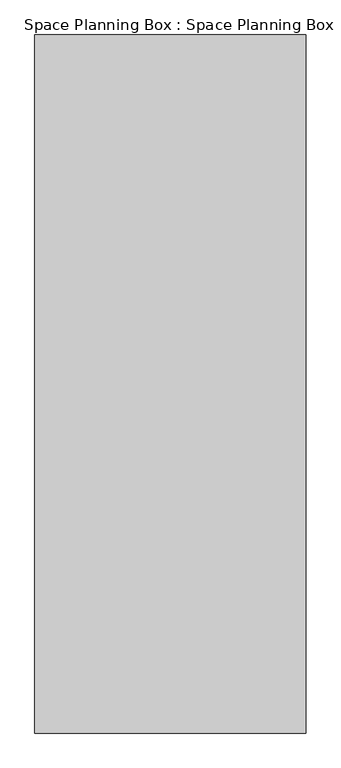
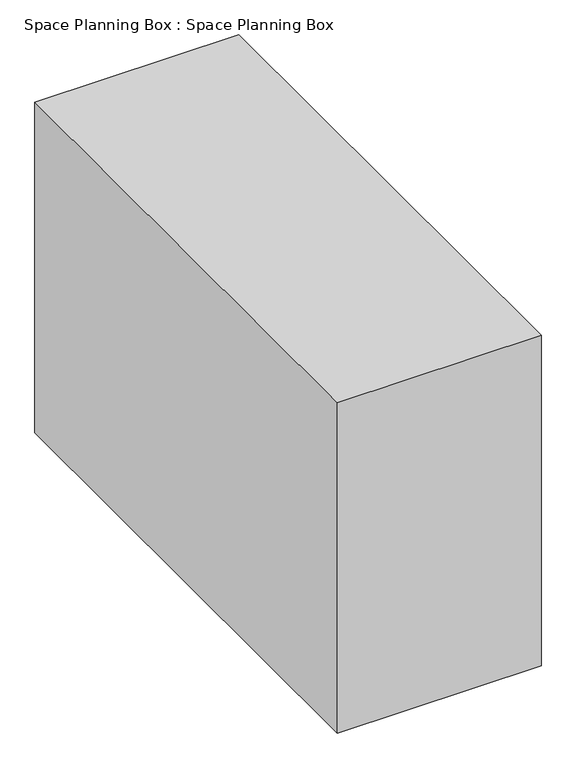
"""IFC4 building model written with IfcOpenShell, lengths in millimetres: proxy geometry, Space Planning Box : Space Planning Box."""

from ifc_helpers import new_model, si_unit, origin, origin_with_axes, place, context, project, spatial, polyline, outline, extrude, source, transform, mapped, element, save


def space_planning_box_space_planning_box_c01b8d6f(model_context):
    return source(origin(), model_context, "Body", "SweptSolid", [
        extrude(outline(polyline([(1750.0, 4500.0), (1750.0, -4500.0), (-1750.0, -4500.0), (-1750.0, 4500.0), (1750.0, 4500.0)])), origin_with_axes(), (0.0, 0.0, 1.0), 6000.0),
    ])


if __name__ == "__main__":
    model = new_model("IFC4")
    model_context = context("Model", 3, world=origin())
    ifc_project = project(units=[si_unit("LENGTHUNIT", "METRE", prefix="MILLI")], contexts=[model_context])
    site = spatial("IfcSite", under=ifc_project)
    building = spatial("IfcBuilding", under=site)
    placement = place(None, origin())
    space_planning_box_space_planning_box_shape = space_planning_box_space_planning_box_c01b8d6f(model_context)
    element("IfcBuildingElementProxy", 1, Name="Space Planning Box : Space Planning Box", ObjectType="Space Planning Box : Space Planning Box", at=placement, inside=building, context=model_context, shape_type="MappedRepresentation", body=[
        mapped(space_planning_box_space_planning_box_shape, transform((0.0, 0.0, 0.0), x_axis=(1.0, 0.0, 0.0), y_axis=(0.0, 1.0, 0.0), z_axis=(0.0, 0.0, 1.0))),
    ])
    save(model, "model.ifc")

# Revit data of these elements
# Type "Space Planning Box : Space Planning Box"
#   Type Comments = "..."
#   Room Name [instance default] = "?"
#   Assembly Code = "..."
#   Width [instance default] = 1524 mm
#   Program Area [instance default] = 0 m²
#   Length [instance default] = 1524 mm
#   Height [instance default] = 1524 mm
#   Area [instance default] = 2.32258 m²
#   Fill Color [instance default] = Cyan
#   Default Elevation = 0
# Element 1 (IfcBuildingElementProxy, "Space Planning Box : Space Planning Box")
#   Room Name = "Kitch & Lunch Room"
#   Width = 3500 mm
#   Program Area = 31.5 m²
#   Length = 9000 mm
#   Height = 6000 mm
#   Area = 31.5 m²
#   Fill Color = Lavender
#   Materials on its faces: "Lavender"
# Materials
#   "Cyan": class "Generic", colour RGB 0 255 255, transparency 0.2, Cost = 0
#   "Lavender": class "Generic", colour RGB 186 85 211, transparency 0.2, Cost = 0
